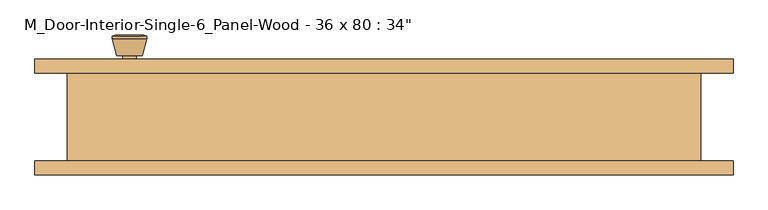
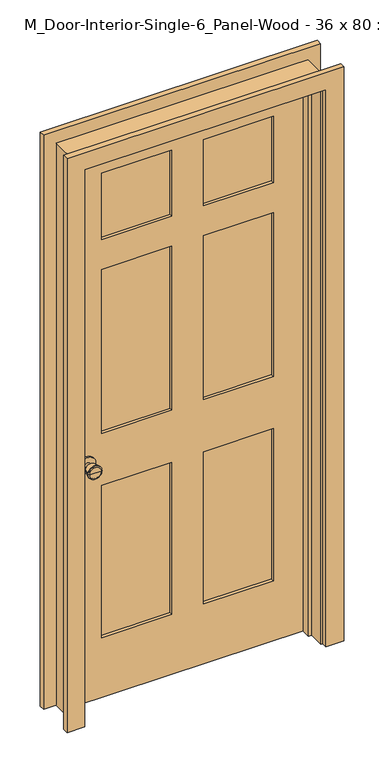
"""IFC4 building model written with IfcOpenShell, lengths in millimetres: door geometry."""

from ifc_helpers import new_model, si_unit, point, frame, frame_2d, origin, place, context, project, spatial, polyline, circle_curve, trimmed, segment, composite_curve, outline, extrude, faceted_brep, source, transform, mapped, element, save
from ifc_brep_helpers import plane_surface, cylinder_surface, revolved_surface, advanced_brep


def door_827a3609(model_context):
    return source(origin(), model_context, "Body", "SolidModel", [
        advanced_brep(
        [(-366.8, 19.325, 914.4), (-356.8, 19.325, 914.4), (-376.8, 19.325, 914.4), (-346.3241324, -29.675, 914.4), (-366.8, -29.675, 914.4), (-387.2758676, -29.675, 914.4), (-341.8, -27.8471319, 914.4), (-391.8, -27.8471319, 914.4), (-341.8, -24.3834537, 914.4), (-391.8, -24.3834537, 914.4), (-348.163764, 0.325, 914.4), (-385.436236, 0.325, 914.4), (-356.8, 0.325, 914.4), (-376.8, 0.325, 914.4)],
        [
            (0, 1),
            (1, 2, circle_curve(frame((-366.8, 19.325, 914.4), z_axis=(0.0, 1.0, 0.0), x_axis=(-1.0, 0.0, 0.0)), 10.0)),
            (2, 0),
            (2, 1, circle_curve(frame((-366.8, 19.325, 914.4), z_axis=(0.0, 1.0, 0.0), x_axis=(-1.0, 0.0, 0.0)), 10.0)),
            (3, 4),
            (4, 5),
            (5, 3, circle_curve(frame((-366.8, -29.675, 914.4), z_axis=(0.0, -1.0, 0.0), x_axis=(-1.0, 0.0, 0.0)), 20.4758676)),
            (3, 5, circle_curve(frame((-366.8, -29.675, 914.4), z_axis=(0.0, -1.0, 0.0), x_axis=(-1.0, 0.0, 0.0)), 20.4758676)),
            (6, 3),
            (5, 7),
            (7, 6, circle_curve(frame((-366.8, -27.8471319, 914.4), z_axis=(0.0, -1.0, 0.0), x_axis=(-1.0, 0.0, 0.0)), 25.0)),
            (6, 7, circle_curve(frame((-366.8, -27.8471319, 914.4), z_axis=(0.0, -1.0, 0.0), x_axis=(-1.0, 0.0, 0.0)), 25.0)),
            (8, 6),
            (7, 9),
            (9, 8, circle_curve(frame((-366.8, -24.3834537, 914.4), z_axis=(0.0, -1.0, 0.0), x_axis=(-1.0, 0.0, 0.0)), 25.0)),
            (8, 9, circle_curve(frame((-366.8, -24.3834537, 914.4), z_axis=(0.0, -1.0, 0.0), x_axis=(-1.0, 0.0, 0.0)), 25.0)),
            (10, 8),
            (9, 11),
            (11, 10, circle_curve(frame((-366.8, 0.325, 914.4), z_axis=(0.0, -1.0, 0.0), x_axis=(-1.0, 0.0, 0.0)), 18.636236)),
            (10, 11, circle_curve(frame((-366.8, 0.325, 914.4), z_axis=(0.0, -1.0, 0.0), x_axis=(-1.0, 0.0, 0.0)), 18.636236)),
            (12, 10),
            (11, 13),
            (13, 12, circle_curve(frame((-366.8, 0.325, 914.4), z_axis=(0.0, -1.0, 0.0), x_axis=(-1.0, 0.0, 0.0)), 10.0)),
            (12, 13, circle_curve(frame((-366.8, 0.325, 914.4), z_axis=(0.0, -1.0, 0.0), x_axis=(-1.0, 0.0, 0.0)), 10.0)),
            (1, 12),
            (13, 2),
        ],
        [
            plane_surface(frame((-366.8, 19.325, 914.4), z_axis=(0.0, 1.0, 0.0), x_axis=(-1.0, 0.0, 0.0))),
            plane_surface(frame((-366.8, -29.675, 914.4), z_axis=(0.0, -1.0, 0.0), x_axis=(-1.0, 0.0, 0.0))),
            revolved_surface(polyline([(-387.2758676, -29.675, 914.4), (-391.8, -27.8471319, 914.4)]), (-366.8, 19.325, 914.4), (0.0, 1.0, 0.0)),
            cylinder_surface(frame((-366.8, 19.325, 914.4), z_axis=(0.0, 1.0, 0.0), x_axis=(-1.0, 0.0, 0.0)), 25.0),
            revolved_surface(polyline([(-391.8, -24.3834537, 914.4), (-385.436236, 0.325, 914.4)]), (-366.8, 19.325, 914.4), (0.0, 1.0, 0.0)),
            plane_surface(frame((-366.8, 0.325, 914.4), z_axis=(0.0, 1.0, 0.0), x_axis=(-1.0, 0.0, 0.0))),
            cylinder_surface(frame((-366.8, 19.325, 914.4), z_axis=(0.0, 1.0, 0.0), x_axis=(-1.0, 0.0, 0.0)), 10.0),
        ],
        [
            (0, [[1, 2, 3]]),
            (0, [[-3, 4, -1]]),
            (1, [[5, 6, 7]]),
            (1, [[-6, -5, 8]]),
            (2, [[9, -7, 10, 11]]),
            (2, [[-10, -8, -9, 12]]),
            (3, [[13, -11, 14, 15]]),
            (3, [[-14, -12, -13, 16]]),
            (4, [[17, -15, 18, 19]]),
            (4, [[-18, -16, -17, 20]]),
            (5, [[21, -19, 22, 23]]),
            (5, [[-22, -20, -21, 24]]),
            (6, [[25, -23, 26, -2]]),
            (6, [[-26, -24, -25, -4]]),
        ],
    ),
        extrude(outline(composite_curve([segment(trimmed(circle_curve(frame_2d((914.4, -366.8)), 30.0), [point((914.4, -396.8))], [point((914.4, -336.8))], False, "CARTESIAN"), True, "CONTINUOUS"), segment(trimmed(circle_curve(frame_2d((914.4, -366.8)), 30.0), [point((914.4, -336.8))], [point((914.4, -396.8))], False, "CARTESIAN"), True, "CONTINUOUS")], self_intersect=False)), frame((0.0, 19.325, 0.0), z_axis=(0.0, 1.0, 0.0), x_axis=(0.0, 0.0, 1.0)), (0.0, 0.0, 1.0), 6.0),
        advanced_brep(
        [(-366.8, 66.325, 914.4), (-376.8, 66.325, 914.4), (-356.8, 66.325, 914.4), (-346.3241324, 115.325, 914.4), (-387.2758676, 115.325, 914.4), (-366.8, 115.325, 914.4), (-341.8, 113.4971319, 914.4), (-391.8, 113.4971319, 914.4), (-341.8, 110.0334537, 914.4), (-391.8, 110.0334537, 914.4), (-348.163764, 85.325, 914.4), (-385.436236, 85.325, 914.4), (-356.8, 85.325, 914.4), (-376.8, 85.325, 914.4)],
        [
            (0, 1),
            (1, 2, circle_curve(frame((-366.8, 66.325, 914.4), z_axis=(0.0, -1.0, 0.0), x_axis=(-1.0, 0.0, 0.0)), 10.0)),
            (2, 0),
            (2, 1, circle_curve(frame((-366.8, 66.325, 914.4), z_axis=(0.0, -1.0, 0.0), x_axis=(-1.0, 0.0, 0.0)), 10.0)),
            (3, 4, circle_curve(frame((-366.8, 115.325, 914.4), z_axis=(0.0, 1.0, 0.0), x_axis=(-1.0, 0.0, 0.0)), 20.4758676)),
            (4, 5),
            (5, 3),
            (4, 3, circle_curve(frame((-366.8, 115.325, 914.4), z_axis=(0.0, 1.0, 0.0), x_axis=(-1.0, 0.0, 0.0)), 20.4758676)),
            (6, 7, circle_curve(frame((-366.8, 113.4971319, 914.4), z_axis=(0.0, 1.0, 0.0), x_axis=(-1.0, 0.0, 0.0)), 25.0)),
            (7, 4),
            (3, 6),
            (7, 6, circle_curve(frame((-366.8, 113.4971319, 914.4), z_axis=(0.0, 1.0, 0.0), x_axis=(-1.0, 0.0, 0.0)), 25.0)),
            (8, 9, circle_curve(frame((-366.8, 110.0334537, 914.4), z_axis=(0.0, 1.0, 0.0), x_axis=(-1.0, 0.0, 0.0)), 25.0)),
            (9, 7),
            (6, 8),
            (9, 8, circle_curve(frame((-366.8, 110.0334537, 914.4), z_axis=(0.0, 1.0, 0.0), x_axis=(-1.0, 0.0, 0.0)), 25.0)),
            (10, 11, circle_curve(frame((-366.8, 85.325, 914.4), z_axis=(0.0, 1.0, 0.0), x_axis=(-1.0, 0.0, 0.0)), 18.636236)),
            (11, 9),
            (8, 10),
            (11, 10, circle_curve(frame((-366.8, 85.325, 914.4), z_axis=(0.0, 1.0, 0.0), x_axis=(-1.0, 0.0, 0.0)), 18.636236)),
            (12, 13, circle_curve(frame((-366.8, 85.325, 914.4), z_axis=(0.0, 1.0, 0.0), x_axis=(-1.0, 0.0, 0.0)), 10.0)),
            (13, 11),
            (10, 12),
            (13, 12, circle_curve(frame((-366.8, 85.325, 914.4), z_axis=(0.0, 1.0, 0.0), x_axis=(-1.0, 0.0, 0.0)), 10.0)),
            (1, 13),
            (12, 2),
        ],
        [
            plane_surface(frame((-366.8, 66.325, 914.4), z_axis=(0.0, -1.0, 0.0), x_axis=(-1.0, 0.0, 0.0))),
            plane_surface(frame((-366.8, 115.325, 914.4), z_axis=(0.0, 1.0, 0.0), x_axis=(-1.0, 0.0, 0.0))),
            revolved_surface(polyline([(-387.2758676, 115.325, 914.4), (-391.8, 113.4971319, 914.4)]), (-366.8, 66.325, 914.4), (0.0, -1.0, 0.0)),
            cylinder_surface(frame((-366.8, 66.325, 914.4), z_axis=(0.0, -1.0, 0.0), x_axis=(-1.0, 0.0, 0.0)), 25.0),
            revolved_surface(polyline([(-391.8, 110.0334537, 914.4), (-385.436236, 85.325, 914.4)]), (-366.8, 66.325, 914.4), (0.0, -1.0, 0.0)),
            plane_surface(frame((-366.8, 85.325, 914.4), z_axis=(0.0, -1.0, 0.0), x_axis=(-1.0, 0.0, 0.0))),
            cylinder_surface(frame((-366.8, 66.325, 914.4), z_axis=(0.0, -1.0, 0.0), x_axis=(-1.0, 0.0, 0.0)), 10.0),
        ],
        [
            (0, [[1, 2, 3]]),
            (0, [[-3, 4, -1]]),
            (1, [[5, 6, 7]]),
            (1, [[8, -7, -6]]),
            (2, [[9, 10, -5, 11]]),
            (2, [[12, -11, -8, -10]]),
            (3, [[13, 14, -9, 15]]),
            (3, [[16, -15, -12, -14]]),
            (4, [[17, 18, -13, 19]]),
            (4, [[20, -19, -16, -18]]),
            (5, [[21, 22, -17, 23]]),
            (5, [[24, -23, -20, -22]]),
            (6, [[-2, 25, -21, 26]]),
            (6, [[-4, -26, -24, -25]]),
        ],
    ),
        extrude(outline(composite_curve([segment(trimmed(circle_curve(frame_2d((914.4, -366.8)), 30.0), [point((914.4, -396.8))], [point((914.4, -336.8))], False, "CARTESIAN"), True, "CONTINUOUS"), segment(trimmed(circle_curve(frame_2d((914.4, -366.8)), 30.0), [point((914.4, -336.8))], [point((914.4, -396.8))], False, "CARTESIAN"), True, "CONTINUOUS")], self_intersect=False)), frame((0.0, 60.325, 0.0), z_axis=(0.0, 1.0, 0.0), x_axis=(0.0, 0.0, 1.0)), (0.0, 0.0, 1.0), 6.0),
        extrude(outline(polyline([(311.8, 36.9916667), (57.5, 36.9916667), (57.5, 48.6583333), (311.8, 48.6583333), (311.8, 36.9916667)])), frame((0.0, 0.0, 1759.3), z_axis=(0.0, 0.0, 1.0), x_axis=(1.0, 0.0, 0.0)), (0.0, 0.0, 1.0), 254.3),
        extrude(outline(polyline([(311.8, 36.9916667), (57.5, 36.9916667), (57.5, 48.6583333), (311.8, 48.6583333), (311.8, 36.9916667)])), frame((0.0, 0.0, 1014.4), z_axis=(0.0, 0.0, 1.0), x_axis=(1.0, 0.0, 0.0)), (0.0, 0.0, 1.0), 629.9),
        extrude(outline(polyline([(-57.5, 36.9916667), (-311.8, 36.9916667), (-311.8, 48.6583333), (-57.5, 48.6583333), (-57.5, 36.9916667)])), frame((0.0, 0.0, 1014.4), z_axis=(0.0, 0.0, 1.0), x_axis=(1.0, 0.0, 0.0)), (0.0, 0.0, 1.0), 629.9),
        extrude(outline(polyline([(-57.5, 36.9916667), (-311.8, 36.9916667), (-311.8, 48.6583333), (-57.5, 48.6583333), (-57.5, 36.9916667)])), frame((0.0, 0.0, 1759.3), z_axis=(0.0, 0.0, 1.0), x_axis=(1.0, 0.0, 0.0)), (0.0, 0.0, 1.0), 254.3),
        extrude(outline(polyline([(311.8, 36.9916667), (57.5, 36.9916667), (57.5, 48.6583333), (311.8, 48.6583333), (311.8, 36.9916667)])), frame((0.0, 0.0, 230.0), z_axis=(0.0, 0.0, 1.0), x_axis=(1.0, 0.0, 0.0)), (0.0, 0.0, 1.0), 584.4),
        extrude(outline(polyline([(-57.5, 36.9916667), (-311.8, 36.9916667), (-311.8, 48.6583333), (-57.5, 48.6583333), (-57.5, 36.9916667)])), frame((0.0, 0.0, 230.0), z_axis=(0.0, 0.0, 1.0), x_axis=(1.0, 0.0, 0.0)), (0.0, 0.0, 1.0), 584.4),
        extrude(outline(polyline([(2133.6, -431.8), (0.0, -431.8), (0.0, 431.8), (2133.6, 431.8), (2133.6, -431.8)]), holes=[polyline([(2013.6, 57.5), (2013.6, 311.8), (1759.3, 311.8), (1759.3, 57.5), (2013.6, 57.5)]), polyline([(1644.3, 311.8), (1014.4, 311.8), (1014.4, 57.5), (1644.3, 57.5), (1644.3, 311.8)]), polyline([(1014.4, -57.5), (1014.4, -311.8), (1644.3, -311.8), (1644.3, -57.5), (1014.4, -57.5)]), polyline([(1759.3, -311.8), (2013.6, -311.8), (2013.6, -57.5), (1759.3, -57.5), (1759.3, -311.8)]), polyline([(814.4, 57.5), (814.4, 311.8), (230.0, 311.8), (230.0, 57.5), (814.4, 57.5)]), polyline([(230.0, -57.5), (230.0, -311.8), (814.4, -311.8), (814.4, -57.5), (230.0, -57.5)])]), frame((0.0, 25.325, 0.0), z_axis=(0.0, 1.0, 0.0), x_axis=(0.0, 0.0, 1.0)), (0.0, 0.0, 1.0), 35.0),
        faceted_brep([(456.8, 60.325, 0.0), (456.8, -66.675, 0.0), (431.8, -66.675, 0.0), (431.8, -9.6, 0.0), (419.1, -9.6, 0.0), (419.1, 25.325, 0.0), (431.8, 25.325, 0.0), (431.8, 60.325, 0.0), (456.8, 60.325, 2158.6), (456.8, -66.675, 2158.6), (-456.8, -66.675, 2158.6), (-456.8, -66.675, 0.0), (-431.8, -66.675, 0.0), (-431.8, -66.675, 2133.6), (431.8, -66.675, 2133.6), (431.8, -9.6, 2133.6), (-431.8, -9.6, 2133.6), (-431.8, -9.6, 0.0), (-419.1, -9.6, 0.0), (-419.1, -9.6, 2120.9), (419.1, -9.6, 2120.9), (419.1, 25.325, 2120.9), (-419.1, 25.325, 2120.9), (-419.1, 25.325, 0.0), (-431.8, 25.325, 0.0), (-431.8, 25.325, 2133.6), (431.8, 25.325, 2133.6), (431.8, 60.325, 2133.6), (-431.8, 60.325, 2133.6), (-431.8, 60.325, 0.0), (-456.8, 60.325, 0.0), (-456.8, 60.325, 2158.6)], [[[0, 1, 2, 3, 4, 5, 6, 7]], [[1, 0, 8, 9]], [[2, 1, 9, 10, 11, 12, 13, 14]], [[3, 2, 14, 15]], [[4, 3, 15, 16, 17, 18, 19, 20]], [[5, 4, 20, 21]], [[6, 5, 21, 22, 23, 24, 25, 26]], [[7, 6, 26, 27]], [[0, 7, 27, 28, 29, 30, 31, 8]], [[9, 8, 31, 10]], [[15, 14, 13, 16]], [[21, 20, 19, 22]], [[27, 26, 25, 28]], [[30, 29, 24, 23, 18, 17, 12, 11]], [[10, 31, 30, 11]], [[16, 13, 12, 17]], [[22, 19, 18, 23]], [[28, 25, 24, 29]]]),
        extrude(outline(polyline([(0.0, 438.15), (0.0, 503.15), (2204.95, 503.15), (2204.95, -503.15), (0.0, -503.15), (0.0, -438.15), (2139.95, -438.15), (2139.95, 438.15), (0.0, 438.15)])), frame((0.0, -86.675, 0.0), z_axis=(0.0, 1.0, 0.0), x_axis=(0.0, 0.0, 1.0)), (0.0, 0.0, 1.0), 20.0),
        extrude(outline(polyline([(0.0, 438.15), (0.0, 503.15), (2204.95, 503.15), (2204.95, -503.15), (0.0, -503.15), (0.0, -438.15), (2139.95, -438.15), (2139.95, 438.15), (0.0, 438.15)])), frame((0.0, 60.325, 0.0), z_axis=(0.0, 1.0, 0.0), x_axis=(0.0, 0.0, 1.0)), (0.0, 0.0, 1.0), 20.0),
    ])


if __name__ == "__main__":
    model = new_model("IFC4")
    model_context = context("Model", 3, world=origin())
    ifc_project = project(units=[si_unit("LENGTHUNIT", "METRE", prefix="MILLI")], contexts=[model_context])
    site = spatial("IfcSite", under=ifc_project)
    building = spatial("IfcBuilding", under=site)
    placement = place(None, origin())
    door_shape = door_827a3609(model_context)
    element("IfcDoor", 1, ObjectType="M_Door-Interior-Single-6_Panel-Wood - 36 x 80 : 34\"", at=placement, inside=building, context=model_context, shape_type="MappedRepresentation", body=[
        mapped(door_shape, transform((0.0, 0.0, 0.0), x_axis=(1.0, 0.0, 0.0), y_axis=(0.0, 1.0, 0.0), z_axis=(0.0, 0.0, 1.0))),
    ])
    save(model, "model.ifc")

# Revit data of these elements
# Type "M_Door-Interior-Single-6_Panel-Wood - 36 x 80 : 34\""
#   Type Mark = "t"
#   Assembly Code = "C1020300"
#   Analytic Construction = "Wooden"
#   Top Rail = 0' - 4.72441"
#   Top Panel = 0' - 10.01181"
#   Thickness = 0' - 1.37795"
#   Thermal Resistance (R) = 0.455703 (m²·K)/W
#   Swing Angle [instance default] = 90.00°
#   Stiles = 0' - 4.72441"
#   Rough Width = 2' - 11.9685"
#   Rough Height = 7' - 0.98425"
#   Mullion = 0' - 4.52756"
#   Lock Rail = 0' - 7.87402"
#   Intermediate Rail = 0' - 4.52756"
#   Height = 7' - 0"
#   Width = 2' - 10"
#   Heat Transfer Coefficient (U) = 2.19465 W/(m²·K)
#   Bottom Rail = 0' - 9.05512"
#   Trim Material = Trim
#   Panel Material = Trim
#   Frame Material = Trim
#   Door Handle Material = Aluminum
#   Visual Light Transmittance = 0
#   Solar Heat Gain Coefficient = 0
#   Wall Closure = (empty or 0)
#   Function = (empty or 0)
# Element 1 (IfcDoor, "M_Door-Interior-Single-6_Panel-Wood - 36 x 80 : 34\"")
#   Materials on its faces: "Trim", "Aluminum"
# Materials
#   "Trim": class "Wood", colour RGB 250 251 245, transparency 0, Cost = 0
#   "Aluminum": class "Metal", colour RGB 244 244 244, transparency 0, Description = "Aluminum 6061", Cost = 0
